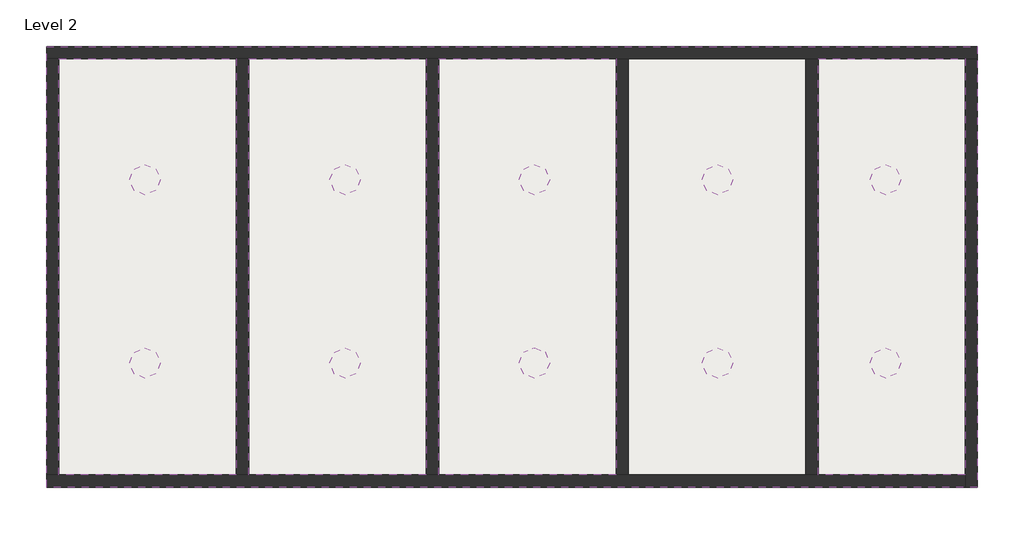
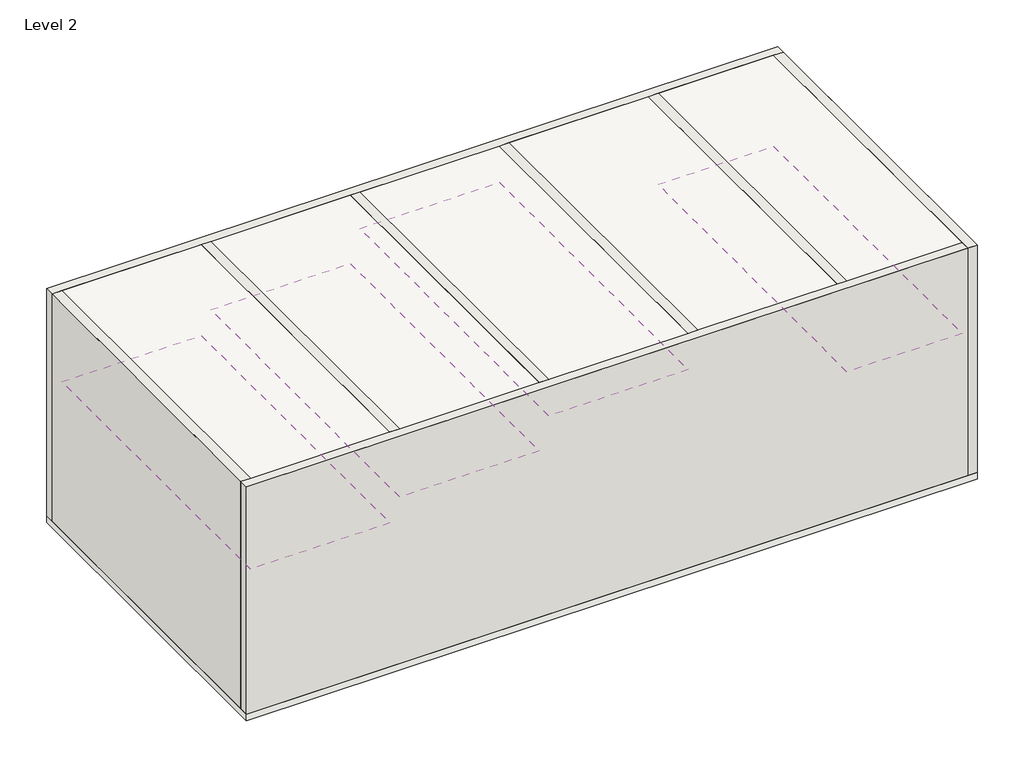
# One storey: 10 light fixtures, 8 walls, 4 coverings, 2 slabs.
"""IFC4 building model written with IfcOpenShell, lengths in millimetres."""

import ifcopenshell
import ifcopenshell.guid

model = None  # the IFC model being written
_history = None  # IfcOwnerHistory: only IFC2X3 demands one
_inside = {}  # id of a spatial element -> (the spatial element, [elements in it])
_under = {}  # id of a project, library or spatial element -> (it, [spatial elements below it])
_declared = {}  # id of a project -> (the project, [libraries it declares])
_typed = {}  # id of a type object -> (the type object, [elements of that type])
_made_of = {}  # id of a material, layer set ... -> (it, [elements and type objects made of it])


def new_model(schema):
    """Start an empty IFC model of exactly this schema.

    Asked for "IFC4X3", IfcOpenShell would pick the latest addendum, in which some entities
    have other attributes; the version numbers below select the first issue.
    IFC2X3 requires an IfcOwnerHistory on every rooted entity: one is made here for all.
    """
    global model, _history
    if schema == "IFC4X3":
        model = ifcopenshell.file(schema_version=(4, 3, 0, 0))
    else:
        model = ifcopenshell.file(schema=schema)
    _inside.clear()
    _under.clear()
    _declared.clear()
    _typed.clear()
    _made_of.clear()
    _history = None
    if model.schema == "IFC2X3":
        org = make("IfcOrganization", Name="unknown")
        user = make(
            "IfcPersonAndOrganization",
            ThePerson=make("IfcPerson", FamilyName="unknown"),
            TheOrganization=org,
        )
        app = make(
            "IfcApplication",
            ApplicationDeveloper=org,
            Version="unknown",
            ApplicationFullName="unknown",
            ApplicationIdentifier="unknown",
        )
        _history = make(
            "IfcOwnerHistory",
            OwningUser=user,
            OwningApplication=app,
            ChangeAction="ADDED",
            CreationDate=0,
        )
    return model


def make(cls, **values):
    """One entity of the class cls with the attributes given. An attribute that is None is left unset."""
    return model.create_entity(
        cls, **{name: value for name, value in values.items() if value is not None}
    )


def rooted(cls, **values):
    """An entity with a GlobalId (a new one), such as an element, a storey or a relation."""
    return make(cls, GlobalId=ifcopenshell.guid.new(), OwnerHistory=_history, **values)


def si_unit(unit_type, name, prefix=None):
    """IfcSIUnit, for example si_unit("LENGTHUNIT", "METRE", prefix="MILLI")."""
    return make("IfcSIUnit", UnitType=unit_type, Prefix=prefix, Name=name)


def assignment(units):
    """IfcUnitAssignment: the units of a project."""
    return None if units is None else make("IfcUnitAssignment", Units=units)


def point(xyz):
    """IfcCartesianPoint."""
    return None if xyz is None else make("IfcCartesianPoint", Coordinates=xyz)


def direction(xyz):
    """IfcDirection."""
    return None if xyz is None else make("IfcDirection", DirectionRatios=xyz)


def frame(location, z_axis=None, x_axis=None):
    """IfcAxis2Placement3D, a coordinate frame: its origin and axes. An axis left out is left unset."""
    return make(
        "IfcAxis2Placement3D",
        Location=point(location),
        Axis=direction(z_axis),
        RefDirection=direction(x_axis),
    )


def frame_2d(location, x_axis=None):
    """IfcAxis2Placement2D, a coordinate frame in the plane: its origin and x axis."""
    return make(
        "IfcAxis2Placement2D", Location=point(location), RefDirection=direction(x_axis)
    )


def origin():
    """The frame at (0, 0, 0) with its axes left unset."""
    return frame((0.0, 0.0, 0.0))


def origin_2d():
    """The frame at (0, 0) in the plane with its x axis left unset."""
    return frame_2d((0.0, 0.0))


def place(relative_to, where):
    """IfcLocalPlacement: puts the frame where relative to a parent placement (None: the world)."""
    return make(
        "IfcLocalPlacement", PlacementRelTo=relative_to, RelativePlacement=where
    )


def context(
    kind, dimensions, precision=None, world=None, true_north=None, identifier=None
):
    """IfcGeometricRepresentationContext, for example the 3D "Model" context."""
    return make(
        "IfcGeometricRepresentationContext",
        ContextIdentifier=identifier,
        ContextType=kind,
        CoordinateSpaceDimension=dimensions,
        Precision=precision,
        WorldCoordinateSystem=world,
        TrueNorth=true_north,
    )


def project(units=None, contexts=None):
    """IfcProject with its units and contexts."""
    return rooted(
        "IfcProject",
        Name="project",
        RepresentationContexts=contexts,
        UnitsInContext=assignment(units),
    )


def spatial(cls, under=None, at=None, **own):
    """A site, building, storey or space (cls), placed at a placement, below another one or the project."""
    s = rooted(cls, ObjectPlacement=at, **own)
    if under is not None:
        _under.setdefault(under.id(), (under, []))[1].append(s)
    return s


def polyline(points):
    """IfcPolyline through the points."""
    return make("IfcPolyline", Points=[point(p) for p in points])


def circle_curve(where, radius):
    """IfcCircle in the frame where."""
    return make("IfcCircle", Position=where, Radius=radius)


def ellipse_curve(where, semi_axis1, semi_axis2):
    """IfcEllipse in the frame where."""
    return make(
        "IfcEllipse", Position=where, SemiAxis1=semi_axis1, SemiAxis2=semi_axis2
    )


def trimmed(basis, trim1, trim2, sense, master):
    """IfcTrimmedCurve: the piece of a basis curve between two trims."""
    return make(
        "IfcTrimmedCurve",
        BasisCurve=basis,
        Trim1=trim1,
        Trim2=trim2,
        SenseAgreement=sense,
        MasterRepresentation=master,
    )


def segment(curve, same_sense, transition):
    """IfcCompositeCurveSegment."""
    return make(
        "IfcCompositeCurveSegment",
        Transition=transition,
        SameSense=same_sense,
        ParentCurve=curve,
    )


def composite_curve(segments, self_intersect=None):
    """IfcCompositeCurve: segments joined end to end."""
    return make("IfcCompositeCurve", Segments=segments, SelfIntersect=self_intersect)


def outline(outer, holes=None, kind="AREA"):
    """IfcArbitraryClosedProfileDef: a profile drawn as a closed curve; with holes, ...WithVoids."""
    if holes is None:
        return make("IfcArbitraryClosedProfileDef", ProfileType=kind, OuterCurve=outer)
    return make(
        "IfcArbitraryProfileDefWithVoids",
        ProfileType=kind,
        OuterCurve=outer,
        InnerCurves=holes,
    )


def extrude(swept, where, along, depth):
    """IfcExtrudedAreaSolid: the profile swept, set in the frame where, extruded along a direction by depth."""
    return make(
        "IfcExtrudedAreaSolid",
        SweptArea=swept,
        Position=where,
        ExtrudedDirection=direction(along),
        Depth=depth,
    )


def faces_of(points, faces, orient=None, outer=None):
    """IfcFace entities. A face is a list of loops; a loop is a list of indices into points, from 0.

    orient and outer hold one flag for each loop. By default every Orientation is true, the
    first loop of a face is its IfcFaceOuterBound and the others are IfcFaceBound.
    """
    made = []
    for i, loops in enumerate(faces):
        bounds = []
        for j, loop in enumerate(loops):
            is_outer = j == 0 if outer is None else outer[i][j]
            bounds.append(
                make(
                    "IfcFaceOuterBound" if is_outer else "IfcFaceBound",
                    Bound=make("IfcPolyLoop", Polygon=[points[k] for k in loop]),
                    Orientation=True if orient is None else orient[i][j],
                )
            )
        made.append(make("IfcFace", Bounds=bounds))
    return made


def faceted_brep(points, faces, orient=None, outer=None, voids=None):
    """IfcFacetedBrep: a solid bounded by flat faces; with voids (closed shells), ...WithVoids."""
    shared = [point(p) for p in points]
    hull = make("IfcClosedShell", CfsFaces=faces_of(shared, faces, orient, outer))
    if voids is None:
        return make("IfcFacetedBrep", Outer=hull)
    return make(
        "IfcFacetedBrepWithVoids",
        Outer=hull,
        Voids=[
            make(cls, CfsFaces=faces_of(shared, fs, o, b)) for cls, fs, o, b in voids
        ],
    )


def shape(context_of_items, identifier, shape_type, items):
    """IfcShapeRepresentation: the items that make up one representation, for example the "Body"."""
    return make(
        "IfcShapeRepresentation",
        ContextOfItems=context_of_items,
        RepresentationIdentifier=identifier,
        RepresentationType=shape_type,
        Items=items,
    )


def source(mapping_origin, context_of_items, identifier, shape_type, items):
    """IfcRepresentationMap: a shape defined once, which mapped items show again and again."""
    return make(
        "IfcRepresentationMap",
        MappingOrigin=mapping_origin,
        MappedRepresentation=shape(context_of_items, identifier, shape_type, items),
    )


def transform(
    local_origin,
    x_axis=None,
    y_axis=None,
    z_axis=None,
    scale=None,
    scale2=None,
    scale3=None,
    uniform=True,
):
    """IfcCartesianTransformationOperator3D, or its non-uniform kind. x_axis, y_axis, z_axis: its Axis1, 2, 3."""
    if uniform:
        return make(
            "IfcCartesianTransformationOperator3D",
            Axis1=direction(x_axis),
            Axis2=direction(y_axis),
            LocalOrigin=point(local_origin),
            Scale=scale,
            Axis3=direction(z_axis),
        )
    return make(
        "IfcCartesianTransformationOperator3DnonUniform",
        Axis1=direction(x_axis),
        Axis2=direction(y_axis),
        LocalOrigin=point(local_origin),
        Scale=scale,
        Axis3=direction(z_axis),
        Scale2=scale2,
        Scale3=scale3,
    )


def mapped(mapping_source, mapping_target):
    """IfcMappedItem: shows the shape of a source again, moved by a transform."""
    return make(
        "IfcMappedItem", MappingSource=mapping_source, MappingTarget=mapping_target
    )


def made_of(thing, what):
    """Note that an element or type object is made of a material, layer set ...; save() writes the relation."""
    if what is not None:
        _made_of.setdefault(what.id(), (what, []))[1].append(thing)
    return thing


def element(
    cls,
    number,
    at=None,
    inside=None,
    cuts=None,
    type_object=None,
    material=None,
    context=None,
    identifier="Body",
    shape_type=None,
    held_by="IfcProductDefinitionShape",
    body=None,
    shapes=None,
    **own,
):
    """One element of the class cls, such as IfcWall. Its Tag is "e" and its number.

    at: its placement. inside: the storey or other place that contains it. cuts: it is an
    opening in that element (IfcRelVoidsElement). A single representation is given by context,
    identifier, shape_type and body (its items); several are given by shapes. held_by: the class
    of the entity that holds the representations. save() writes the other relations.
    """
    e = rooted(cls, Tag="e%d" % number, ObjectPlacement=at, **own)
    if body is not None:
        shapes = [shape(context, identifier, shape_type, body)]
    if shapes is not None:
        e.Representation = make(held_by, Representations=shapes)
    if inside is not None:
        _inside.setdefault(inside.id(), (inside, []))[1].append(e)
    if cuts is not None:
        rooted(
            "IfcRelVoidsElement", RelatingBuildingElement=cuts, RelatedOpeningElement=e
        )
    if type_object is not None:
        _typed.setdefault(type_object.id(), (type_object, []))[1].append(e)
    return made_of(e, material)


def aggregate(whole, parts):
    """IfcRelAggregates: a whole, such as a stair, and the parts it consists of."""
    return rooted("IfcRelAggregates", RelatingObject=whole, RelatedObjects=parts)


def save(model, path):
    """Write the relations noted so far, then the file.

    IfcRelAggregates (storeys below a building ...), IfcRelContainedInSpatialStructure (elements
    in a storey), IfcRelDefinesByType, IfcRelAssociatesMaterial and IfcRelDeclares: one each for
    every whole, place, type object, material and project.
    """
    for whole, parts in _under.values():
        aggregate(whole, parts)
    for where, things in _inside.values():
        rooted(
            "IfcRelContainedInSpatialStructure",
            RelatedElements=things,
            RelatingStructure=where,
        )
    for kind, things in _typed.values():
        rooted("IfcRelDefinesByType", RelatedObjects=things, RelatingType=kind)
    for what, things in _made_of.values():
        rooted("IfcRelAssociatesMaterial", RelatedObjects=things, RelatingMaterial=what)
    for by, libraries in _declared.values():
        rooted("IfcRelDeclares", RelatingContext=by, RelatedDefinitions=libraries)
    model.write(path)


def plane_surface(at):
    """IfcPlane: the flat surface through the origin of the frame at, square to its z axis."""
    return make("IfcPlane", Position=at)


def revolved_surface(curve, axis_point, axis_direction):
    """IfcSurfaceOfRevolution: the curve turned about the line through axis_point along axis_direction."""
    return make(
        "IfcSurfaceOfRevolution",
        SweptCurve=make("IfcArbitraryOpenProfileDef", ProfileType="CURVE", Curve=curve),
        AxisPosition=make("IfcAxis1Placement", Location=point(axis_point), Axis=direction(axis_direction)),
    )


def advanced_brep(points, edges, surfaces, faces):
    """IfcAdvancedBrep: a solid bounded by faces that lie on surfaces and meet in shared edges.

    An edge is (start, end): straight between two places in points (the first is 0);
    or (start, end, curve); or (start, end, curve, False) where it runs against its curve.
    A face is (place in surfaces, loops), or (place, loops, False) where it looks against
    its surface's normal. A loop lists edges by number (the first is 1), with a minus sign
    where the edge is run from its end to its start. The first loop is the outer one.
    """
    corners = [point(p) for p in points]
    vertices = [make("IfcVertexPoint", VertexGeometry=c) for c in corners]
    made = []
    for start, end, *more in edges:
        made.append(
            make(
                "IfcEdgeCurve",
                EdgeStart=vertices[start],
                EdgeEnd=vertices[end],
                EdgeGeometry=more[0] if more else make("IfcPolyline", Points=[corners[start], corners[end]]),
                SameSense=more[1] if len(more) > 1 else True,
            )
        )
    hull = []
    for where, loops, *sense in faces:
        bounds = []
        for j, loop in enumerate(loops):
            ring = [make("IfcOrientedEdge", EdgeElement=made[abs(k) - 1], Orientation=k > 0) for k in loop]
            bounds.append(
                make(
                    "IfcFaceOuterBound" if j == 0 else "IfcFaceBound",
                    Bound=make("IfcEdgeLoop", EdgeList=ring),
                    Orientation=True,
                )
            )
        hull.append(make("IfcAdvancedFace", Bounds=bounds, FaceSurface=surfaces[where], SameSense=sense[0] if sense else True))
    return make("IfcAdvancedBrep", Outer=make("IfcClosedShell", CfsFaces=hull))


def downlight_downlight_e6a68a7d(model_context):
    return source(origin(), model_context, "Body", "SolidModel", [
        advanced_brep(
        [(-230.0, 0.0, 0.0), (230.0, 0.0, 0.0), (0.0, 0.0, 0.0), (0.0, 0.0, 70.3180567)],
        [
            (0, 1, circle_curve(frame((0.0, 0.0, 0.0), z_axis=(0.0, 0.0, -1.0), x_axis=(1.0, 0.0, 0.0)), 230.0)),
            (1, 2),
            (2, 0),
            (1, 0, circle_curve(frame((0.0, 0.0, 0.0), z_axis=(0.0, 0.0, -1.0), x_axis=(1.0, 0.0, 0.0)), 230.0)),
            (3, 1, circle_curve(frame((13.1969865, 0.0, -297.8236248), z_axis=(0.0, 1.0, 0.0), x_axis=(1.0, 0.0, 0.0)), 368.3781456)),
            (0, 3, circle_curve(frame((-13.1969865, 0.0, -297.8236248), z_axis=(0.0, 1.0, 0.0), x_axis=(-1.0, 0.0, 0.0)), 368.3781456)),
        ],
        [
            plane_surface(frame((0.0, 0.0, 0.0), z_axis=(0.0, 0.0, -1.0), x_axis=(1.0, 0.0, 0.0))),
            revolved_surface(trimmed(ellipse_curve(frame((13.1969865, 0.0, -297.8236248), z_axis=(0.0, -1.0, 0.0), x_axis=(1.0, 0.0, 0.0)), 368.3781456, 368.3781456), [point((230.0, 0.0, 0.0))], [point((0.0, 0.0, 70.3180567))], True, "CARTESIAN"), (0.0, 0.0, 2194.0651339), (0.0, 0.0, 1.0)),
        ],
        [
            (0, [[1, 2, 3]]),
            (0, [[4, -3, -2]]),
            (1, [[5, -1, 6]]),
            (1, [[-6, -4, -5]]),
        ],
    ),
        extrude(outline(composite_curve([segment(trimmed(circle_curve(origin_2d(), 250.0), [point((-250.0, 0.0))], [point((250.0, 0.0))], False, "CARTESIAN"), True, "CONTINUOUS"), segment(trimmed(circle_curve(origin_2d(), 250.0), [point((250.0, 0.0))], [point((-250.0, 0.0))], False, "CARTESIAN"), True, "CONTINUOUS")], self_intersect=False)), frame((0.0, 0.0, -10.1537533), z_axis=(0.0, 0.0, 1.0), x_axis=(1.0, 0.0, 0.0)), (0.0, 0.0, 1.0), 10.1537533),
    ])


model = new_model("IFC4")

# Units and contexts
model_context = context("Model", 3, world=origin())
ifc_project = project(units=[si_unit("LENGTHUNIT", "METRE", prefix="MILLI")], contexts=[model_context])

# Site, building, storey
site = spatial("IfcSite", under=ifc_project)
building = spatial("IfcBuilding", under=site)
storey = spatial("IfcBuildingStorey", under=building, Name="Level 2", Elevation=5000.0)

# Coverings
placement = place(None, origin())
element("IfcCovering", 1, ObjectType="Plain", at=placement, inside=storey, context=model_context, shape_type="SweptSolid", body=[
    extrude(outline(polyline([(4711.6370984, -2494.7382368), (4711.6370984, 4305.2617632), (7111.6370984, 4305.2617632), (7111.6370984, -2494.7382368), (4711.6370984, -2494.7382368)])), frame((0.0, 0.0, 8000.0), z_axis=(0.0, 0.0, 1.0), x_axis=(1.0, 0.0, 0.0)), (0.0, 0.0, 1.0), 57.0),
])
element("IfcCovering", 2, ObjectType="Plain", at=placement, inside=storey, context=model_context, shape_type="SweptSolid", body=[
    extrude(outline(polyline([(-1488.3629016, -2494.7382368), (-1488.3629016, 4305.2617632), (1411.6370984, 4305.2617632), (1411.6370984, -2494.7382368), (-1488.3629016, -2494.7382368)])), frame((0.0, 0.0, 9200.0), z_axis=(0.0, 0.0, 1.0), x_axis=(1.0, 0.0, 0.0)), (0.0, 0.0, 1.0), 57.0),
])
element("IfcCovering", 3, ObjectType="Plain", at=placement, inside=storey, context=model_context, shape_type="SweptSolid", body=[
    extrude(outline(polyline([(-4588.3629016, -2494.7382368), (-4588.3629016, 4305.2617632), (-1688.3629016, 4305.2617632), (-1688.3629016, -2494.7382368), (-4588.3629016, -2494.7382368)])), frame((0.0, 0.0, 8500.0), z_axis=(0.0, 0.0, 1.0), x_axis=(1.0, 0.0, 0.0)), (0.0, 0.0, 1.0), 57.0),
])
element("IfcCovering", 4, ObjectType="Plain", at=placement, inside=storey, context=model_context, shape_type="SweptSolid", body=[
    extrude(outline(polyline([(-7688.3629016, 4305.2617632), (-4788.3629016, 4305.2617632), (-4788.3629016, -2494.7382368), (-7688.3629016, -2494.7382368), (-7688.3629016, 4305.2617632)])), frame((0.0, 0.0, 8000.0), z_axis=(0.0, 0.0, 1.0), x_axis=(1.0, 0.0, 0.0)), (0.0, 0.0, 1.0), 57.0),
])

# Light fixtures
downlight_downlight_shape = downlight_downlight_e6a68a7d(model_context)
element("IfcLightFixture", 5, ObjectType="Downlight : Downlight", at=placement, inside=storey, context=model_context, shape_type="MappedRepresentation", body=[
    mapped(downlight_downlight_shape, transform((-6281.2033206, -666.9973068, 8000.0), x_axis=(1.0, 0.0, 0.0), y_axis=(0.0, 1.0, 0.0), z_axis=(0.0, 0.0, 1.0))),
])
element("IfcLightFixture", 6, ObjectType="Downlight : Downlight", at=placement, inside=storey, context=model_context, shape_type="MappedRepresentation", body=[
    mapped(downlight_downlight_shape, transform((-6281.2033206, 2328.2026932, 8000.0), x_axis=(1.0, 0.0, 0.0), y_axis=(0.0, 1.0, 0.0), z_axis=(0.0, 0.0, 1.0))),
])
element("IfcLightFixture", 7, ObjectType="Downlight : Downlight", at=placement, inside=storey, context=model_context, shape_type="MappedRepresentation", body=[
    mapped(downlight_downlight_shape, transform((-3013.7777439, -666.9973068, 8500.0), x_axis=(1.0, 0.0, 0.0), y_axis=(0.0, 1.0, 0.0), z_axis=(0.0, 0.0, 1.0))),
])
element("IfcLightFixture", 8, ObjectType="Downlight : Downlight", at=placement, inside=storey, context=model_context, shape_type="MappedRepresentation", body=[
    mapped(downlight_downlight_shape, transform((-3013.7777439, 2328.2026932, 8500.0), x_axis=(1.0, 0.0, 0.0), y_axis=(0.0, 1.0, 0.0), z_axis=(0.0, 0.0, 1.0))),
])
element("IfcLightFixture", 9, ObjectType="Downlight : Downlight", at=placement, inside=storey, context=model_context, shape_type="MappedRepresentation", body=[
    mapped(downlight_downlight_shape, transform((76.5388311, -666.9973068, 9200.0), x_axis=(1.0, 0.0, 0.0), y_axis=(0.0, 1.0, 0.0), z_axis=(0.0, 0.0, 1.0))),
])
element("IfcLightFixture", 10, ObjectType="Downlight : Downlight", at=placement, inside=storey, context=model_context, shape_type="MappedRepresentation", body=[
    mapped(downlight_downlight_shape, transform((76.5388311, 2328.2026932, 9200.0), x_axis=(1.0, 0.0, 0.0), y_axis=(0.0, 1.0, 0.0), z_axis=(0.0, 0.0, 1.0))),
])
element("IfcLightFixture", 11, ObjectType="Downlight : Downlight", at=placement, inside=storey, context=model_context, shape_type="MappedRepresentation", body=[
    mapped(downlight_downlight_shape, transform((3067.3545284, -666.9973068, 8900.0), x_axis=(1.0, 0.0, 0.0), y_axis=(0.0, 1.0, 0.0), z_axis=(0.0, 0.0, 1.0))),
])
element("IfcLightFixture", 12, ObjectType="Downlight : Downlight", at=placement, inside=storey, context=model_context, shape_type="MappedRepresentation", body=[
    mapped(downlight_downlight_shape, transform((3067.3545284, 2328.2026932, 8900.0), x_axis=(1.0, 0.0, 0.0), y_axis=(0.0, 1.0, 0.0), z_axis=(0.0, 0.0, 1.0))),
])
element("IfcLightFixture", 13, ObjectType="Downlight : Downlight", at=placement, inside=storey, context=model_context, shape_type="MappedRepresentation", body=[
    mapped(downlight_downlight_shape, transform((5810.7393139, -666.9973068, 8000.0), x_axis=(1.0, 0.0, 0.0), y_axis=(0.0, 1.0, 0.0), z_axis=(0.0, 0.0, 1.0))),
])
element("IfcLightFixture", 14, ObjectType="Downlight : Downlight", at=placement, inside=storey, context=model_context, shape_type="MappedRepresentation", body=[
    mapped(downlight_downlight_shape, transform((5810.7393139, 2328.2026932, 8000.0), x_axis=(1.0, 0.0, 0.0), y_axis=(0.0, 1.0, 0.0), z_axis=(0.0, 0.0, 1.0))),
])

# Slabs
element("IfcSlab", 15, ObjectType="Generic 150mm", at=placement, inside=storey, context=model_context, shape_type="SweptSolid", body=[
    extrude(outline(polyline([(7311.6370984, 4505.2617632), (7311.6370984, -2694.7382368), (-7888.3629016, -2694.7382368), (-7888.3629016, 4505.2617632), (7311.6370984, 4505.2617632)])), frame((0.0, 0.0, 4850.0), z_axis=(0.0, 0.0, 1.0), x_axis=(1.0, 0.0, 0.0)), (0.0, 0.0, 1.0), 150.0),
])
element("IfcSlab", 16, ObjectType="Generic 150mm", at=placement, inside=storey, context=model_context, shape_type="SweptSolid", body=[
    extrude(outline(polyline([(7311.6370984, 4505.2617632), (7311.6370984, -2694.7382368), (-7888.3629016, -2694.7382368), (-7888.3629016, 4505.2617632), (7311.6370984, 4505.2617632)])), frame((0.0, 0.0, 9850.0), z_axis=(0.0, 0.0, 1.0), x_axis=(1.0, 0.0, 0.0)), (0.0, 0.0, 1.0), 150.0),
])

# Walls
element("IfcWall", 17, ObjectType="Generic - 200mm", at=placement, inside=storey, context=model_context, shape_type="Brep", body=[
    faceted_brep([(-7888.3629016, 4305.2617632, 5000.0), (-7688.3629016, 4305.2617632, 5000.0), (-4788.3629016, 4305.2617632, 5000.0), (-4588.3629016, 4305.2617632, 5000.0), (-1688.3629016, 4305.2617632, 5000.0), (-1488.3629016, 4305.2617632, 5000.0), (1411.6370984, 4305.2617632, 5000.0), (1611.6370984, 4305.2617632, 5000.0), (4511.6370984, 4305.2617632, 5000.0), (4711.6370984, 4305.2617632, 5000.0), (7111.6370984, 4305.2617632, 5000.0), (7311.6370984, 4305.2617632, 5000.0), (7311.6370984, 4305.2617632, 10000.0), (7111.6370984, 4305.2617632, 10000.0), (4711.6370984, 4305.2617632, 10000.0), (4511.6370984, 4305.2617632, 10000.0), (1611.6370984, 4305.2617632, 10000.0), (1411.6370984, 4305.2617632, 10000.0), (-1488.3629016, 4305.2617632, 10000.0), (-1688.3629016, 4305.2617632, 10000.0), (-4588.3629016, 4305.2617632, 10000.0), (-4788.3629016, 4305.2617632, 10000.0), (-7688.3629016, 4305.2617632, 10000.0), (-7888.3629016, 4305.2617632, 10000.0), (-7888.3629016, 4505.2617632, 5000.0), (-7888.3629016, 4505.2617632, 10000.0), (7311.6370984, 4505.2617632, 10000.0), (7311.6370984, 4505.2617632, 5000.0)], [[[0, 1, 2, 3, 4, 5, 6, 7, 8, 9, 10, 11, 12, 13, 14, 15, 16, 17, 18, 19, 20, 21, 22, 23]], [[24, 25, 26, 27]], [[11, 10, 9, 8, 7, 6, 5, 4, 3, 2, 1, 0, 24, 27]], [[23, 22, 21, 20, 19, 18, 17, 16, 15, 14, 13, 12, 26, 25]], [[12, 11, 27, 26]], [[0, 23, 25, 24]]]),
])
element("IfcWall", 18, ObjectType="Generic - 200mm", at=placement, inside=storey, context=model_context, shape_type="Brep", body=[
    faceted_brep([(7111.6370984, 4305.2617632, 5000.0), (7111.6370984, -2494.7382368, 5000.0), (7111.6370984, -2694.7382368, 5000.0), (7111.6370984, -2694.7382368, 10000.0), (7111.6370984, -2494.7382368, 10000.0), (7111.6370984, 4305.2617632, 10000.0), (7311.6370984, 4305.2617632, 5000.0), (7311.6370984, 4305.2617632, 10000.0), (7311.6370984, -2694.7382368, 10000.0), (7311.6370984, -2694.7382368, 5000.0)], [[[0, 1, 2, 3, 4, 5]], [[6, 7, 8, 9]], [[2, 1, 0, 6, 9]], [[5, 4, 3, 8, 7]], [[0, 5, 7, 6]], [[3, 2, 9, 8]]]),
])
element("IfcWall", 19, ObjectType="Generic - 200mm", at=placement, inside=storey, context=model_context, shape_type="Brep", body=[
    faceted_brep([(7111.6370984, -2494.7382368, 5000.0), (4711.6370984, -2494.7382368, 5000.0), (4511.6370984, -2494.7382368, 5000.0), (1611.6370984, -2494.7382368, 5000.0), (1411.6370984, -2494.7382368, 5000.0), (-1488.3629016, -2494.7382368, 5000.0), (-1688.3629016, -2494.7382368, 5000.0), (-4588.3629016, -2494.7382368, 5000.0), (-4788.3629016, -2494.7382368, 5000.0), (-7688.3629016, -2494.7382368, 5000.0), (-7888.3629016, -2494.7382368, 5000.0), (-7888.3629016, -2494.7382368, 10000.0), (-7688.3629016, -2494.7382368, 10000.0), (-4788.3629016, -2494.7382368, 10000.0), (-4588.3629016, -2494.7382368, 10000.0), (-1688.3629016, -2494.7382368, 10000.0), (-1488.3629016, -2494.7382368, 10000.0), (1411.6370984, -2494.7382368, 10000.0), (1611.6370984, -2494.7382368, 10000.0), (4511.6370984, -2494.7382368, 10000.0), (4711.6370984, -2494.7382368, 10000.0), (7111.6370984, -2494.7382368, 10000.0), (7111.6370984, -2694.7382368, 5000.0), (7111.6370984, -2694.7382368, 10000.0), (-7888.3629016, -2694.7382368, 10000.0), (-7888.3629016, -2694.7382368, 5000.0)], [[[0, 1, 2, 3, 4, 5, 6, 7, 8, 9, 10, 11, 12, 13, 14, 15, 16, 17, 18, 19, 20, 21]], [[22, 23, 24, 25]], [[10, 9, 8, 7, 6, 5, 4, 3, 2, 1, 0, 22, 25]], [[21, 20, 19, 18, 17, 16, 15, 14, 13, 12, 11, 24, 23]], [[0, 21, 23, 22]], [[11, 10, 25, 24]]]),
])
element("IfcWall", 20, ObjectType="Generic - 200mm", at=placement, inside=storey, context=model_context, shape_type="SweptSolid", body=[
    extrude(outline(polyline([(-7688.3629016, 4305.2617632), (-7688.3629016, -2494.7382368), (-7888.3629016, -2494.7382368), (-7888.3629016, 4305.2617632), (-7688.3629016, 4305.2617632)])), frame((0.0, 0.0, 5000.0), z_axis=(0.0, 0.0, 1.0), x_axis=(1.0, 0.0, 0.0)), (0.0, 0.0, 1.0), 5000.0),
])
element("IfcWall", 21, ObjectType="Generic - 200mm", at=placement, inside=storey, context=model_context, shape_type="SweptSolid", body=[
    extrude(outline(polyline([(-4788.3629016, -2494.7382368), (-4788.3629016, 4305.2617632), (-4588.3629016, 4305.2617632), (-4588.3629016, -2494.7382368), (-4788.3629016, -2494.7382368)])), frame((0.0, 0.0, 5000.0), z_axis=(0.0, 0.0, 1.0), x_axis=(1.0, 0.0, 0.0)), (0.0, 0.0, 1.0), 5000.0),
])
element("IfcWall", 22, ObjectType="Generic - 200mm", at=placement, inside=storey, context=model_context, shape_type="SweptSolid", body=[
    extrude(outline(polyline([(-1688.3629016, -2494.7382368), (-1688.3629016, 4305.2617632), (-1488.3629016, 4305.2617632), (-1488.3629016, -2494.7382368), (-1688.3629016, -2494.7382368)])), frame((0.0, 0.0, 5000.0), z_axis=(0.0, 0.0, 1.0), x_axis=(1.0, 0.0, 0.0)), (0.0, 0.0, 1.0), 5000.0),
])
element("IfcWall", 23, ObjectType="Generic - 200mm", at=placement, inside=storey, context=model_context, shape_type="SweptSolid", body=[
    extrude(outline(polyline([(1411.6370984, -2494.7382368), (1411.6370984, 4305.2617632), (1611.6370984, 4305.2617632), (1611.6370984, -2494.7382368), (1411.6370984, -2494.7382368)])), frame((0.0, 0.0, 5000.0), z_axis=(0.0, 0.0, 1.0), x_axis=(1.0, 0.0, 0.0)), (0.0, 0.0, 1.0), 5000.0),
])
element("IfcWall", 24, ObjectType="Generic - 200mm", at=placement, inside=storey, context=model_context, shape_type="SweptSolid", body=[
    extrude(outline(polyline([(4511.6370984, -2494.7382368), (4511.6370984, 4305.2617632), (4711.6370984, 4305.2617632), (4711.6370984, -2494.7382368), (4511.6370984, -2494.7382368)])), frame((0.0, 0.0, 5000.0), z_axis=(0.0, 0.0, 1.0), x_axis=(1.0, 0.0, 0.0)), (0.0, 0.0, 1.0), 5000.0),
])

save(model, "model.ifc")

# Revit data of these elements
# Type "Plain"
#   built-in parameter 1002203 = 1 (stored number, unit not read)
#   built-in parameter 1002202 = 1 (stored number, unit not read)
#   Layers, outside or top first: 0.045 m "Metal Stud Layer" (function 1); 0.012 m "Gypsum Wall Board" (function 1)
# Type "Downlight : Downlight"
#   Default Elevation = 0
# Type "Generic 150mm"
#   Function = 0
#   Layers, outside or top first: 0.15 m no material (function 1)
# Type "Generic - 200mm"
#   Layers, outside or top first: 0.2 m no material (function 1)
# Elements 1, 4 (IfcCovering, "Plain")
#   Height Offset From Level = 3 m
#   Phase Created = New Construction
#   Materials on its faces: "Gypsum Wall Board", "Metal Stud Layer"
# Element 2 (IfcCovering, "Plain")
#   Height Offset From Level = 4.2 m
#   Phase Created = New Construction
#   Materials on its faces: "Gypsum Wall Board", "Metal Stud Layer"
# Element 3 (IfcCovering, "Plain")
#   Height Offset From Level = 3.5 m
#   Phase Created = New Construction
#   Materials on its faces: "Gypsum Wall Board", "Metal Stud Layer"
# Element 5 (IfcLightFixture, "Downlight : Downlight")
#   Mark = "45"
#   Phase Created = New Construction
# Element 6 (IfcLightFixture, "Downlight : Downlight")
#   Mark = "46"
#   Phase Created = New Construction
# Element 7 (IfcLightFixture, "Downlight : Downlight")
#   Mark = "47"
#   Phase Created = New Construction
# Element 8 (IfcLightFixture, "Downlight : Downlight")
#   Mark = "48"
#   Phase Created = New Construction
# Element 9 (IfcLightFixture, "Downlight : Downlight")
#   Mark = "49"
#   Phase Created = New Construction
# Element 10 (IfcLightFixture, "Downlight : Downlight")
#   Mark = "50"
#   Phase Created = New Construction
# Element 11 (IfcLightFixture, "Downlight : Downlight")
#   Mark = "51"
#   Phase Created = New Construction
# Element 12 (IfcLightFixture, "Downlight : Downlight")
#   Mark = "52"
#   Phase Created = New Construction
# Element 13 (IfcLightFixture, "Downlight : Downlight")
#   Mark = "53"
#   Phase Created = New Construction
# Element 14 (IfcLightFixture, "Downlight : Downlight")
#   Mark = "54"
#   Phase Created = New Construction
# Element 15 (IfcSlab, "Generic 150mm")
#   Height Offset From Level = 0 m
#   Phase Created = New Construction
#   Materials on its faces: "Default Floor"
# Element 16 (IfcSlab, "Generic 150mm")
#   Height Offset From Level = 5 m
#   Phase Created = New Construction
#   Materials on its faces: "Default Floor"
# Elements 17, 18, 19, 20, 21, 22, 23, 24 (IfcWall, "Generic - 200mm")
#   Top Offset = 5 m
#   Base Offset = 0 m
#   wall height = 5 m
#   Phase Created = New Construction
#   Base Constraint = Level 2
#   Top Constraint = Level 2
#   Materials on its faces: "Default Wall"
# Materials
#   "Metal Stud Layer": class "Metal", colour RGB 127 127 127, transparency 0, Description = "Light gauge steel framing, thermal air layer", Cost = 0
#   "Gypsum Wall Board": class "Generic", colour RGB 249 249 249, transparency 0, Description = "Gypsum Wall Board", Cost = 0
#   "Default Floor": class "Miscellaneous", colour RGB 127 127 127, transparency 0, Cost = 0
#   "Default Wall": class "Miscellaneous", colour RGB 128 128 128, transparency 0, Cost = 0
